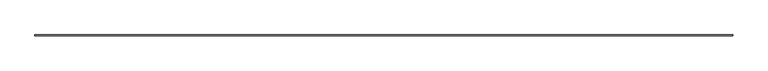
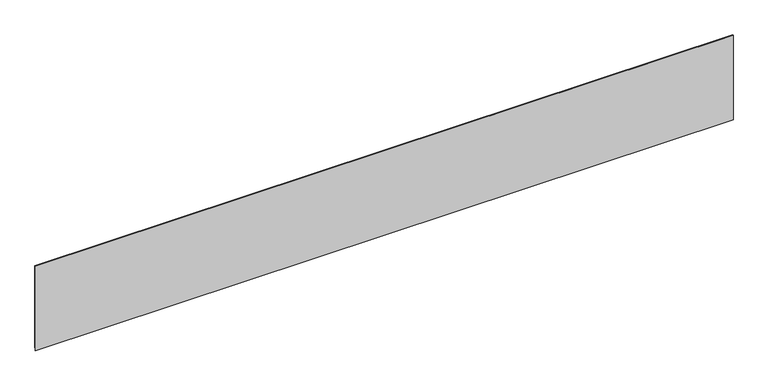
"""IFC4 building model written with IfcOpenShell, lengths in millimetres: proxy geometry, Generic Models 7:Generic Models 1:5:Generic Models 1:5 : Generic Models 7:Generic Models 1:337419:14 : Generic Models 7:Generic Models 1:5:Generic Models 1:5 : Generic Models 7:Generic Models 1:337419:311462."""

from ifc_helpers import new_model, si_unit, frame, origin, place, context, project, spatial, polyline, outline, extrude, source, transform, mapped, element, save


def generic_models_9de1f82b(model_context):
    return source(origin(), model_context, "Body", "SweptSolid", [
        extrude(outline(polyline([(-579029.0720892, 3723.834699), (-579038.7913841, 3723.834699), (-579038.7913841, 6155.090949), (-579019.7413841, 6155.090949), (-579019.7413841, 3795.8780043), (-579029.0720892, 3784.758103), (-579029.0720892, 3723.834699)])), frame((560327.5617239, 0.0, 0.0), z_axis=(1.0, 0.0, 0.0), x_axis=(0.0, 1.0, 0.0)), (0.0, 0.0, 1.0), 19018.2500001),
    ])


if __name__ == "__main__":
    model = new_model("IFC4")
    model_context = context("Model", 3, world=origin())
    ifc_project = project(units=[si_unit("LENGTHUNIT", "METRE", prefix="MILLI")], contexts=[model_context])
    site = spatial("IfcSite", under=ifc_project)
    building = spatial("IfcBuilding", under=site)
    placement = place(None, origin())
    generic_models_shape = generic_models_9de1f82b(model_context)
    element("IfcBuildingElementProxy", 1, Name="Generic Models 7:Generic Models 1:5:Generic Models 1:5 : Generic Models 7:Generic Models 1:337419:14 : Generic Models 7:Generic Models 1:5:Generic Models 1:5 : Generic Models 7:Generic Models 1:337419:311462", ObjectType="Generic Models 7:Generic Models 1:5:Generic Models 1:5 : Generic Models 7:Generic Models 1:337419:14 : Generic Models 7:Generic Models 1:5:Generic Models 1:5 : Generic Models 7:Generic Models 1:337419:311462", at=placement, inside=building, context=model_context, shape_type="MappedRepresentation", body=[
        mapped(generic_models_shape, transform((0.0, 0.0, 0.0), x_axis=(1.0, 0.0, 0.0), y_axis=(0.0, 1.0, 0.0), z_axis=(0.0, 0.0, 1.0))),
    ])
    save(model, "model.ifc")

# Revit data of these elements
# Type "Generic Models 7:Generic Models 1:5:Generic Models 1:5 : Generic Models 7:Generic Models 1:337419:14 : Generic Models 7:Generic Models 1:5:Generic Models 1:5 : Generic Models 7:Generic Models 1:337419:311462"
#   NameOverride = "Generic Models 7:Generic Models 1:5:Generic Models 1:5 : Generic Models 7:Generic Models 1:337419:311462"
#   ObjectTypeOverride = "Generic Models 1:5 : Generic Models 7:Generic Models 1:337419"
#   Reference = "Generic Models 1"
#   Tag = "311462"
# Element 1 (IfcBuildingElementProxy, "Generic Models 7:Generic Models 1:5:Generic Models 1:5 : Generic Models 7:Generic Models 1:337419:14 : Generic Models 7:Generic Models 1:5:Generic Models 1:5 : Generic Models 7:Generic Models 1:337419:311462")
#   Materials on its faces: "1\" MINERAL WOOL BOARD INSULATION"
# Materials
#   "1\" MINERAL WOOL BOARD INSULATION": class "Unassigned", colour RGB 205 188 106, transparency 0, Cost = 0
